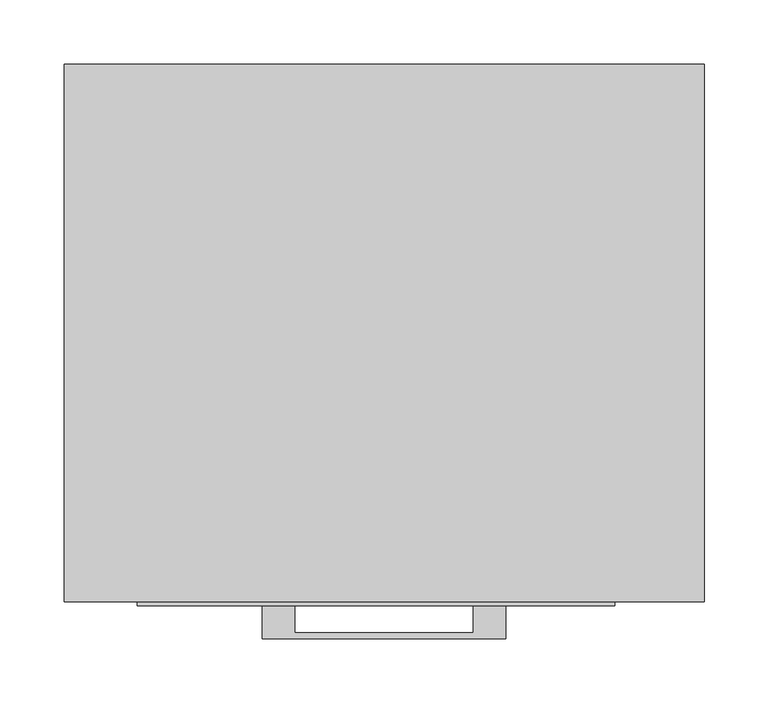
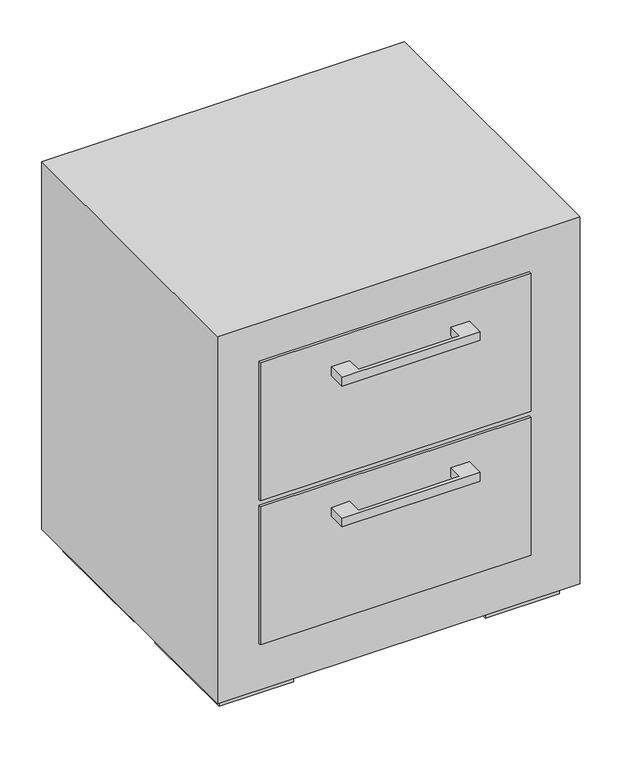
"""IFC4 building model written with IfcOpenShell, lengths in millimetres: furniture geometry, Criado mudo : Criado mudo."""

import ifcopenshell
import ifcopenshell.guid

model = None  # the IFC model being written
_history = None  # IfcOwnerHistory: only IFC2X3 demands one
_inside = {}  # id of a spatial element -> (the spatial element, [elements in it])
_under = {}  # id of a project, library or spatial element -> (it, [spatial elements below it])
_declared = {}  # id of a project -> (the project, [libraries it declares])
_typed = {}  # id of a type object -> (the type object, [elements of that type])
_made_of = {}  # id of a material, layer set ... -> (it, [elements and type objects made of it])


def new_model(schema):
    """Start an empty IFC model of exactly this schema.

    Asked for "IFC4X3", IfcOpenShell would pick the latest addendum, in which some entities
    have other attributes; the version numbers below select the first issue.
    IFC2X3 requires an IfcOwnerHistory on every rooted entity: one is made here for all.
    """
    global model, _history
    if schema == "IFC4X3":
        model = ifcopenshell.file(schema_version=(4, 3, 0, 0))
    else:
        model = ifcopenshell.file(schema=schema)
    _inside.clear()
    _under.clear()
    _declared.clear()
    _typed.clear()
    _made_of.clear()
    _history = None
    if model.schema == "IFC2X3":
        org = make("IfcOrganization", Name="unknown")
        user = make(
            "IfcPersonAndOrganization",
            ThePerson=make("IfcPerson", FamilyName="unknown"),
            TheOrganization=org,
        )
        app = make(
            "IfcApplication",
            ApplicationDeveloper=org,
            Version="unknown",
            ApplicationFullName="unknown",
            ApplicationIdentifier="unknown",
        )
        _history = make(
            "IfcOwnerHistory",
            OwningUser=user,
            OwningApplication=app,
            ChangeAction="ADDED",
            CreationDate=0,
        )
    return model


def make(cls, **values):
    """One entity of the class cls with the attributes given. An attribute that is None is left unset."""
    return model.create_entity(
        cls, **{name: value for name, value in values.items() if value is not None}
    )


def rooted(cls, **values):
    """An entity with a GlobalId (a new one), such as an element, a storey or a relation."""
    return make(cls, GlobalId=ifcopenshell.guid.new(), OwnerHistory=_history, **values)


def si_unit(unit_type, name, prefix=None):
    """IfcSIUnit, for example si_unit("LENGTHUNIT", "METRE", prefix="MILLI")."""
    return make("IfcSIUnit", UnitType=unit_type, Prefix=prefix, Name=name)


def assignment(units):
    """IfcUnitAssignment: the units of a project."""
    return None if units is None else make("IfcUnitAssignment", Units=units)


def point(xyz):
    """IfcCartesianPoint."""
    return None if xyz is None else make("IfcCartesianPoint", Coordinates=xyz)


def direction(xyz):
    """IfcDirection."""
    return None if xyz is None else make("IfcDirection", DirectionRatios=xyz)


def frame(location, z_axis=None, x_axis=None):
    """IfcAxis2Placement3D, a coordinate frame: its origin and axes. An axis left out is left unset."""
    return make(
        "IfcAxis2Placement3D",
        Location=point(location),
        Axis=direction(z_axis),
        RefDirection=direction(x_axis),
    )


def origin():
    """The frame at (0, 0, 0) with its axes left unset."""
    return frame((0.0, 0.0, 0.0))


def origin_with_axes():
    """The frame at (0, 0, 0) with the z axis (0, 0, 1) and the x axis (1, 0, 0) written out."""
    return frame((0.0, 0.0, 0.0), z_axis=(0.0, 0.0, 1.0), x_axis=(1.0, 0.0, 0.0))


def place(relative_to, where):
    """IfcLocalPlacement: puts the frame where relative to a parent placement (None: the world)."""
    return make(
        "IfcLocalPlacement", PlacementRelTo=relative_to, RelativePlacement=where
    )


def context(
    kind, dimensions, precision=None, world=None, true_north=None, identifier=None
):
    """IfcGeometricRepresentationContext, for example the 3D "Model" context."""
    return make(
        "IfcGeometricRepresentationContext",
        ContextIdentifier=identifier,
        ContextType=kind,
        CoordinateSpaceDimension=dimensions,
        Precision=precision,
        WorldCoordinateSystem=world,
        TrueNorth=true_north,
    )


def project(units=None, contexts=None):
    """IfcProject with its units and contexts."""
    return rooted(
        "IfcProject",
        Name="project",
        RepresentationContexts=contexts,
        UnitsInContext=assignment(units),
    )


def spatial(cls, under=None, at=None, **own):
    """A site, building, storey or space (cls), placed at a placement, below another one or the project."""
    s = rooted(cls, ObjectPlacement=at, **own)
    if under is not None:
        _under.setdefault(under.id(), (under, []))[1].append(s)
    return s


def polyline(points):
    """IfcPolyline through the points."""
    return make("IfcPolyline", Points=[point(p) for p in points])


def outline(outer, holes=None, kind="AREA"):
    """IfcArbitraryClosedProfileDef: a profile drawn as a closed curve; with holes, ...WithVoids."""
    if holes is None:
        return make("IfcArbitraryClosedProfileDef", ProfileType=kind, OuterCurve=outer)
    return make(
        "IfcArbitraryProfileDefWithVoids",
        ProfileType=kind,
        OuterCurve=outer,
        InnerCurves=holes,
    )


def extrude(swept, where, along, depth):
    """IfcExtrudedAreaSolid: the profile swept, set in the frame where, extruded along a direction by depth."""
    return make(
        "IfcExtrudedAreaSolid",
        SweptArea=swept,
        Position=where,
        ExtrudedDirection=direction(along),
        Depth=depth,
    )


def shape(context_of_items, identifier, shape_type, items):
    """IfcShapeRepresentation: the items that make up one representation, for example the "Body"."""
    return make(
        "IfcShapeRepresentation",
        ContextOfItems=context_of_items,
        RepresentationIdentifier=identifier,
        RepresentationType=shape_type,
        Items=items,
    )


def source(mapping_origin, context_of_items, identifier, shape_type, items):
    """IfcRepresentationMap: a shape defined once, which mapped items show again and again."""
    return make(
        "IfcRepresentationMap",
        MappingOrigin=mapping_origin,
        MappedRepresentation=shape(context_of_items, identifier, shape_type, items),
    )


def transform(
    local_origin,
    x_axis=None,
    y_axis=None,
    z_axis=None,
    scale=None,
    scale2=None,
    scale3=None,
    uniform=True,
):
    """IfcCartesianTransformationOperator3D, or its non-uniform kind. x_axis, y_axis, z_axis: its Axis1, 2, 3."""
    if uniform:
        return make(
            "IfcCartesianTransformationOperator3D",
            Axis1=direction(x_axis),
            Axis2=direction(y_axis),
            LocalOrigin=point(local_origin),
            Scale=scale,
            Axis3=direction(z_axis),
        )
    return make(
        "IfcCartesianTransformationOperator3DnonUniform",
        Axis1=direction(x_axis),
        Axis2=direction(y_axis),
        LocalOrigin=point(local_origin),
        Scale=scale,
        Axis3=direction(z_axis),
        Scale2=scale2,
        Scale3=scale3,
    )


def mapped(mapping_source, mapping_target):
    """IfcMappedItem: shows the shape of a source again, moved by a transform."""
    return make(
        "IfcMappedItem", MappingSource=mapping_source, MappingTarget=mapping_target
    )


def made_of(thing, what):
    """Note that an element or type object is made of a material, layer set ...; save() writes the relation."""
    if what is not None:
        _made_of.setdefault(what.id(), (what, []))[1].append(thing)
    return thing


def element(
    cls,
    number,
    at=None,
    inside=None,
    cuts=None,
    type_object=None,
    material=None,
    context=None,
    identifier="Body",
    shape_type=None,
    held_by="IfcProductDefinitionShape",
    body=None,
    shapes=None,
    **own,
):
    """One element of the class cls, such as IfcWall. Its Tag is "e" and its number.

    at: its placement. inside: the storey or other place that contains it. cuts: it is an
    opening in that element (IfcRelVoidsElement). A single representation is given by context,
    identifier, shape_type and body (its items); several are given by shapes. held_by: the class
    of the entity that holds the representations. save() writes the other relations.
    """
    e = rooted(cls, Tag="e%d" % number, ObjectPlacement=at, **own)
    if body is not None:
        shapes = [shape(context, identifier, shape_type, body)]
    if shapes is not None:
        e.Representation = make(held_by, Representations=shapes)
    if inside is not None:
        _inside.setdefault(inside.id(), (inside, []))[1].append(e)
    if cuts is not None:
        rooted(
            "IfcRelVoidsElement", RelatingBuildingElement=cuts, RelatedOpeningElement=e
        )
    if type_object is not None:
        _typed.setdefault(type_object.id(), (type_object, []))[1].append(e)
    return made_of(e, material)


def aggregate(whole, parts):
    """IfcRelAggregates: a whole, such as a stair, and the parts it consists of."""
    return rooted("IfcRelAggregates", RelatingObject=whole, RelatedObjects=parts)


def save(model, path):
    """Write the relations noted so far, then the file.

    IfcRelAggregates (storeys below a building ...), IfcRelContainedInSpatialStructure (elements
    in a storey), IfcRelDefinesByType, IfcRelAssociatesMaterial and IfcRelDeclares: one each for
    every whole, place, type object, material and project.
    """
    for whole, parts in _under.values():
        aggregate(whole, parts)
    for where, things in _inside.values():
        rooted(
            "IfcRelContainedInSpatialStructure",
            RelatedElements=things,
            RelatingStructure=where,
        )
    for kind, things in _typed.values():
        rooted("IfcRelDefinesByType", RelatedObjects=things, RelatingType=kind)
    for what, things in _made_of.values():
        rooted("IfcRelAssociatesMaterial", RelatedObjects=things, RelatingMaterial=what)
    for by, libraries in _declared.values():
        rooted("IfcRelDeclares", RelatingContext=by, RelatedDefinitions=libraries)
    model.write(path)


def furniture_79364497(model_context):
    return source(origin(), model_context, "Body", "SweptSolid", [
        extrude(outline(polyline([(-135.8627073, -12.7), (-135.8627073, -182.0169665), (-238.2627073, -182.0169665), (-238.2627073, -12.7), (-135.8627073, -12.7)])), origin_with_axes(), (0.0, 0.0, 1.0), 14.9168536),
        extrude(outline(polyline([(234.8846936, -12.7), (234.8846936, -182.0169665), (125.1934917, -182.0169665), (125.1934917, -12.7), (234.8846936, -12.7)])), origin_with_axes(), (0.0, 0.0, 1.0), 14.9168536),
        extrude(outline(polyline([(-135.8627073, -232.8169665), (-135.8627073, -385.2169665), (-238.2627073, -385.2169665), (-238.2627073, -232.8169665), (-135.8627073, -232.8169665)])), origin_with_axes(), (0.0, 0.0, 1.0), 14.9168536),
        extrude(outline(polyline([(231.5448501, -232.8169665), (231.5448501, -385.2169665), (129.2372927, -385.2169665), (129.2372927, -232.8169665), (231.5448501, -232.8169665)])), origin_with_axes(), (0.0, 0.0, 1.0), 14.9168536),
        extrude(outline(polyline([(182.5, -401.0919665), (-190.5, -401.0919665), (-190.5, -397.9169665), (182.5, -397.9169665), (182.5, -401.0919665)])), frame((0.0, 0.0, 292.55), z_axis=(0.0, 0.0, 1.0), x_axis=(1.0, 0.0, 0.0)), (0.0, 0.0, 1.0), 201.6125),
        extrude(outline(polyline([(-92.9, -427.0311125), (-92.9, -401.6311125), (-67.5, -401.6311125), (-67.5, -422.2686125), (72.2, -422.2686125), (72.2, -401.6311125), (97.6, -401.6311125), (97.6, -427.0311125), (-92.9, -427.0311125)])), frame((0.0, 0.0, 236.3666599), z_axis=(0.0, 0.0, 1.0), x_axis=(1.0, 0.0, 0.0)), (0.0, 0.0, 1.0), 12.7),
        extrude(outline(polyline([(-92.9, -427.0311125), (-92.9, -401.6311125), (-67.5, -401.6311125), (-67.5, -422.2686125), (72.2, -422.2686125), (72.2, -401.6311125), (97.6, -401.6311125), (97.6, -427.0311125), (-92.9, -427.0311125)])), frame((0.0, 0.0, 441.3666599), z_axis=(0.0, 0.0, 1.0), x_axis=(1.0, 0.0, 0.0)), (0.0, 0.0, 1.0), 12.7),
        extrude(outline(polyline([(182.5, -401.0919665), (-190.5, -401.0919665), (-190.5, -397.9169665), (182.5, -397.9169665), (182.5, -401.0919665)])), frame((0.0, 0.0, 82.55), z_axis=(0.0, 0.0, 1.0), x_axis=(1.0, 0.0, 0.0)), (0.0, 0.0, 1.0), 201.6125),
        extrude(outline(polyline([(252.35, 22.0830335), (252.35, -397.9169665), (-247.65, -397.9169665), (-247.65, 22.0830335), (252.35, 22.0830335)])), frame((0.0, 0.0, 14.9168536), z_axis=(0.0, 0.0, 1.0), x_axis=(1.0, 0.0, 0.0)), (0.0, 0.0, 1.0), 535.0831464),
    ])


if __name__ == "__main__":
    model = new_model("IFC4")
    model_context = context("Model", 3, world=origin())
    ifc_project = project(units=[si_unit("LENGTHUNIT", "METRE", prefix="MILLI")], contexts=[model_context])
    site = spatial("IfcSite", under=ifc_project)
    building = spatial("IfcBuilding", under=site)
    placement = place(None, origin())
    furniture_shape = furniture_79364497(model_context)
    element("IfcFurniture", 1, ObjectType="Criado mudo : Criado mudo", at=placement, inside=building, context=model_context, shape_type="MappedRepresentation", body=[
        mapped(furniture_shape, transform((0.0, 0.0, 0.0), x_axis=(1.0, 0.0, 0.0), y_axis=(0.0, 1.0, 0.0), z_axis=(0.0, 0.0, 1.0))),
    ])
    save(model, "model.ifc")

# Revit data of these elements
# Type "Criado mudo : Criado mudo"
#   Profundidade = 0.42 m
#   Largura = 0.5 m
#   Altura = 0.55 m
#   Material = wood brown
#   Puxador = Handle
#   Default Elevation = 0
# Element 1 (IfcFurniture, "Criado mudo : Criado mudo")
#   Materials on its faces: "wood brown", "Handle"
# Materials
#   "wood brown": class "Wood", colour RGB 80 39 12, transparency 0, Cost = 0
#   "Handle": class "Não atribuído", colour RGB 247 247 247, transparency 0, Cost = 0
